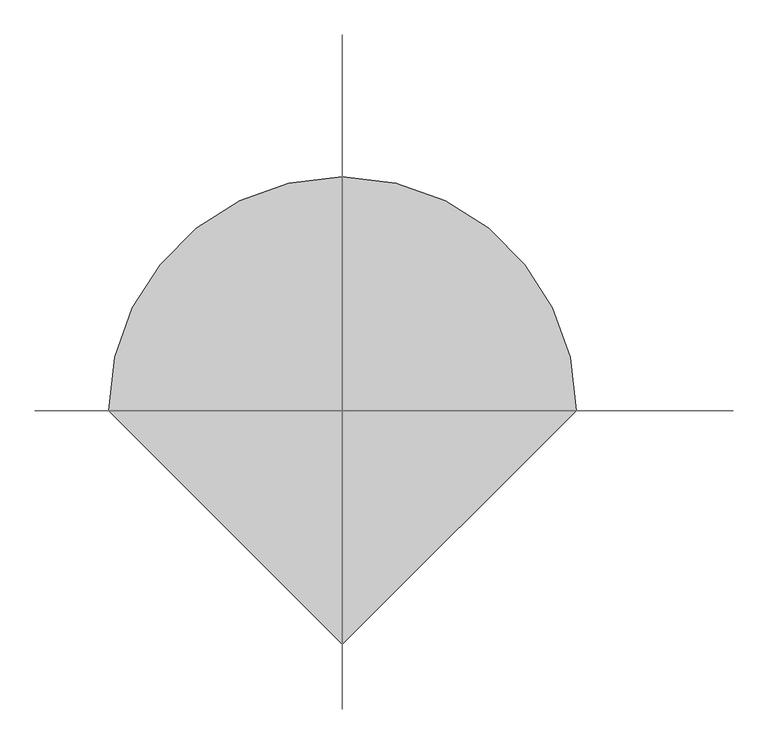
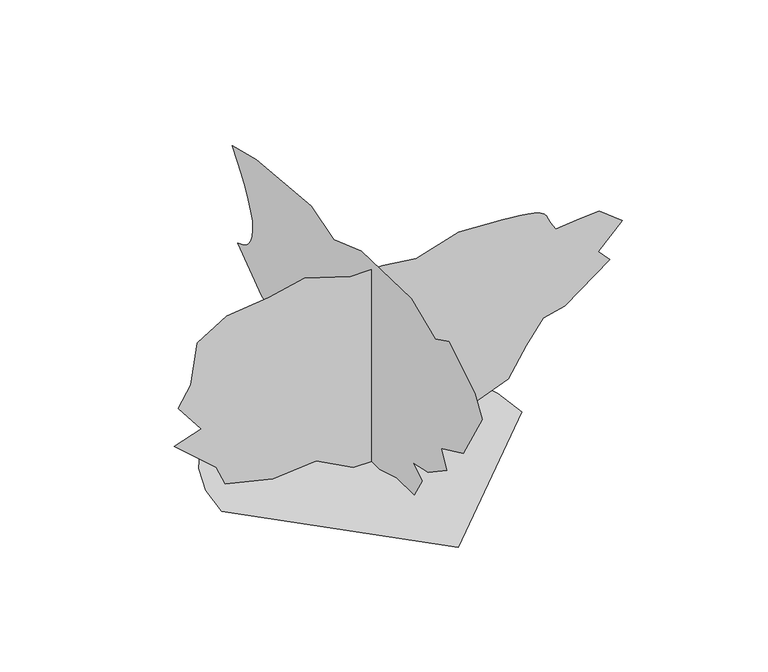
"""IFC4 building model written with IfcOpenShell, lengths in millimetres: proxy geometry, meyer lilac 26082 : meyer lilac 26082."""

from ifc_helpers import new_model, si_unit, origin, place, context, project, spatial, triangles, source, transform, mapped, element, save


def entourage_17e9046c(model_context):
    return source(origin(), model_context, "Body", "Tessellation", [
        triangles([(-84.8149175, -7.75e-05, 8.6e-06), (-258.4957951, -7.39e-05, 93.6967881), (-462.1199759, -8.49e-05, 75.7298434), (-683.7121187, -8.82e-05, 129.6306776), (-725.6373213, -7.86e-05, 225.4544616), (-923.2722055, -6.65e-05, 399.1355936), (-797.5040829, -5.6e-05, 441.0582891), (-905.306805, -4.43e-05, 578.805041), (-845.4161293, -3.03e-05, 674.6290976), (-815.4720268, -5.4e-06, 872.2639091), (-677.7253475, 1.06e-05, 956.1093), (-480.0879198, 2.21e-05, 980.0666313), (-312.397138, 3.37e-05, 1015.9999758), (-96.7927928, 3.53e-05, 950.1199854), (52.9315665, 4.18e-05, 950.1199854), (208.6452405, 4.65e-05, 932.1545849), (406.2806153, 6.23e-05, 992.0452606), (615.896636, 7e-05, 980.0666313), (655.4622442, 7.14e-05, 977.3944834), (693.7171766, 7.27e-05, 974.0950481), (729.355917, 7.37e-05, 969.5382769), (761.0627026, 7.43e-05, 963.0943388), (787.5346333, 7.44e-05, 954.1382721), (807.455801, 7.38e-05, 942.0377026), (819.5208349, 7.25e-05, 926.1652702), (826.871549, 7.08e-05, 909.594334), (833.5949759, 6.94e-05, 895.540468), (839.7925627, 6.83e-05, 883.5796429), (845.5736052, 6.73e-05, 873.2951689), (851.0371525, 6.65e-05, 864.2680309), (856.2924276, 6.57e-05, 856.0790686), (861.443494, 6.5e-05, 848.309194), (975.2355309, 7.14e-05, 860.2852798), (1065.0702364, 7.61e-05, 866.2745945), (1172.8703424, 7.08e-05, 782.4292036), (1059.0809217, 5.23e-05, 668.6397102), (1112.9822828, 4.75e-05, 608.7490708), (903.3662258, 1.97e-05, 453.0343749), (801.5554344, 1.24e-05, 429.0796597), (723.6968147, -3.8e-06, 321.2769739), (639.8513512, -2.39e-05, 183.5315118), (328.4245391, -5.18e-05, 63.7517137), (202.6561802, -5.51e-05, 81.7186584), (100.8435812, -6.93e-05, 5e-07), (0.021362, -58.648346, 1.19e-05), (0.0213578, -202.8161995, 40.9414963), (0.021352, -346.9843074, 46.4863159), (0.021347, -407.9773141, 151.839669), (0.0213581, -335.8946863, 196.1989981), (0.0213523, -457.8832432, 223.9235958), (0.0213509, -607.5959435, 323.7331467), (0.0213526, -563.2348432, 406.9054682), (0.0213517, -740.6741215, 490.0802968), (0.0213453, -895.9316505, 750.6918966), (0.021359, -834.9361004, 844.9538755), (0.0213677, -624.230357, 972.4872248), (0.0213728, -513.3314575, 917.0390104), (0.0213802, -319.2602002, 1000.2113319), (0.0213989, 85.5197618, 989.1216745), (0.0214104, 307.3171429, 911.4942181), (0.0214172, 490.2987428, 966.9424324), (0.021433, 933.8919062, 928.1286678), (0.0214469, 1127.9631998, 878.2227751), (0.0214342, 1091.3973358, 830.7450771), (0.0214336, 1056.4291214, 783.5569691), (0.021433, 1024.6639091, 736.9505116), (0.0214322, 997.699276, 691.2152945), (0.0214311, 977.1354149, 646.6458492), (0.0214298, 964.575135, 603.5319111), (0.0214281, 961.6160133, 562.1629609), (0.0214263, 967.0643726, 525.9679318), (0.0214245, 978.0421909, 497.337085), (0.0214229, 993.625106, 475.0130116), (0.0214213, 1012.893552, 457.7308542), (0.0214197, 1034.9280355, 444.2332769), (0.0214305, 1058.8065926, 433.2554223), (0.021429, 1083.6046429, 423.5399179), (0.0214189, 889.5333492, 279.3720463), (0.0213939, 473.6642567, 135.2049558), (0.021383, 390.489428, 85.3005619), (0.0213686, 124.3337626, 52.0311355), (0.0213699, 41.160192, 0.0), (-701.8553427, 0.0, 8.48e-05), (-683.3005886, 160.8188175, 0.000114), (-630.4584652, 308.5058421, 9.41e-05), (-547.5554223, 438.8281563, 0.0001242), (-438.8281563, 547.5554223, 0.0001065), (-308.5058421, 630.4559217, 9.09e-05), (-160.8188175, 683.3005886, 0.0001273), (3.04e-05, 701.8553427, 0.0001181), (160.8190719, 683.3005886, 0.0001133), (308.5058421, 630.4559217, 0.0001131), (438.8281563, 547.5554223, 0.0001173), (547.5554223, 438.8281563, 0.0001255), (630.4559217, 308.5058421, 8.82e-05), (683.3005886, 160.8188175, 0.0001035), (701.8553427, -6.14e-05, 0.0001219), (-9.28e-05, -701.8553427, 8.86e-05)], [[6, 5, 7], [35, 34, 36], [34, 33, 36], [37, 36, 38], [33, 32, 36], [36, 32, 38], [38, 32, 39], [8, 7, 9], [4, 3, 5], [10, 9, 11], [11, 9, 12], [9, 7, 12], [7, 5, 12], [5, 3, 12], [3, 2, 12], [12, 2, 13], [13, 2, 14], [14, 2, 15], [2, 1, 15], [1, 44, 15], [44, 43, 15], [15, 43, 16], [43, 42, 16], [42, 41, 16], [41, 40, 16], [16, 40, 17], [40, 39, 17], [39, 32, 17], [17, 32, 18], [18, 32, 19], [32, 31, 19], [31, 30, 19], [19, 30, 20], [30, 29, 20], [20, 29, 21], [29, 28, 21], [28, 27, 21], [21, 27, 22], [27, 26, 22], [22, 26, 23], [23, 26, 24], [24, 26, 25], [77, 76, 78], [63, 62, 64], [76, 75, 78], [75, 74, 78], [64, 62, 65], [48, 47, 49], [47, 46, 49], [51, 50, 52], [74, 73, 78], [65, 62, 66], [54, 53, 55], [55, 53, 56], [56, 53, 57], [53, 52, 57], [73, 72, 78], [57, 52, 58], [58, 52, 59], [52, 50, 59], [50, 49, 59], [59, 49, 60], [49, 46, 60], [46, 45, 60], [45, 82, 60], [82, 81, 60], [81, 80, 60], [80, 79, 60], [79, 78, 60], [60, 78, 61], [78, 72, 61], [72, 71, 61], [71, 70, 61], [61, 70, 62], [70, 69, 62], [69, 68, 62], [68, 67, 62], [62, 67, 66], [98, 97, 83], [97, 96, 83], [83, 96, 84], [96, 95, 84], [84, 95, 85], [85, 95, 86], [95, 94, 86], [94, 93, 86], [86, 93, 87], [87, 93, 88], [88, 93, 89], [89, 93, 90], [90, 93, 91], [91, 93, 92]], closed=False),
    ])


if __name__ == "__main__":
    model = new_model("IFC4")
    model_context = context("Model", 3, world=origin())
    ifc_project = project(units=[si_unit("LENGTHUNIT", "METRE", prefix="MILLI")], contexts=[model_context])
    site = spatial("IfcSite", under=ifc_project)
    building = spatial("IfcBuilding", under=site)
    placement = place(None, origin())
    entourage_shape = entourage_17e9046c(model_context)
    element("IfcBuildingElementProxy", 1, Name="meyer lilac 26082 : meyer lilac 26082", ObjectType="meyer lilac 26082 : meyer lilac 26082", at=placement, inside=building, context=model_context, shape_type="MappedRepresentation", body=[
        mapped(entourage_shape, transform((0.0, 0.0, 0.0), x_axis=(1.0, 0.0, 0.0), y_axis=(0.0, 1.0, 0.0), z_axis=(0.0, 0.0, 1.0))),
    ])
    save(model, "model.ifc")

# Revit data of these elements
# Type "meyer lilac 26082 : meyer lilac 26082"
#   built-in parameter 1005195 = "RPC-16-FXGN-2JPX-PG7M-U000-ST1L-LVER-AU"
#   Height = 0
